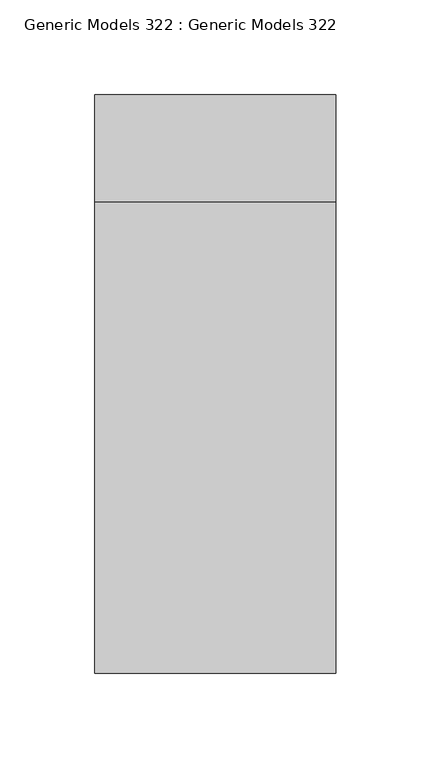
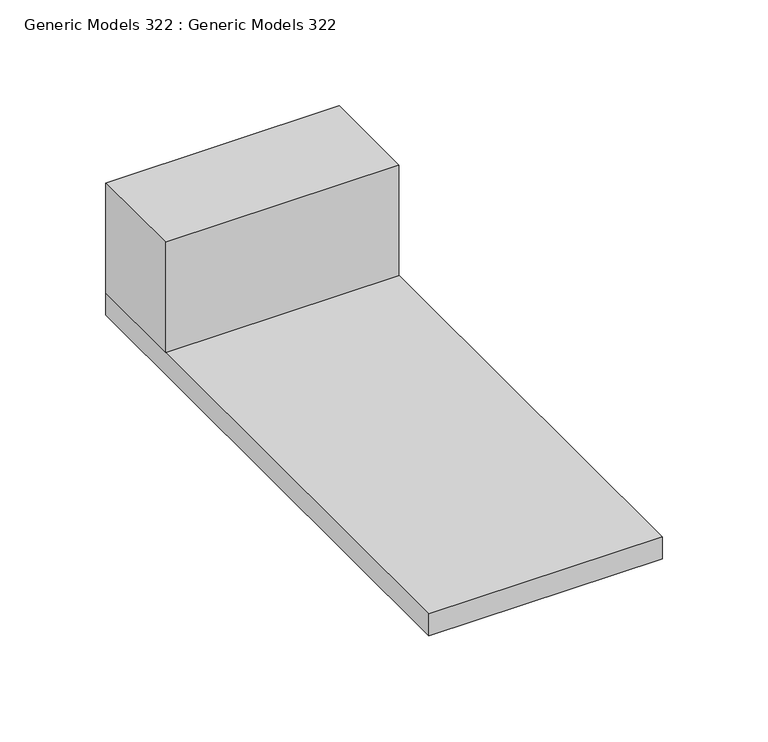
"""IFC4 building model written with IfcOpenShell, lengths in millimetres: proxy geometry, Generic Models 322 : Generic Models 322."""

from ifc_helpers import new_model, si_unit, frame, origin, place, context, project, spatial, polyline, outline, extrude, source, transform, mapped, element, save


def generic_models_322_generic_models_322_8154812b(model_context):
    return source(origin(), model_context, "Body", "SweptSolid", [
        extrude(outline(polyline([(1342.8513704, 704.5309662), (1469.8513704, 704.5309662), (1469.8513704, 648.1582392), (1342.8513704, 648.1582392), (1342.8513704, 704.5309662)])), frame((0.0, 0.0, 123310.396), z_axis=(0.0, 0.0, 1.0), x_axis=(1.0, 0.0, 0.0)), (0.0, 0.0, 1.0), 63.5),
        extrude(outline(polyline([(1342.8513704, 704.5309662), (1469.8513704, 704.5309662), (1469.8513704, 399.7309662), (1342.8513704, 399.7309662), (1342.8513704, 704.5309662)])), frame((0.0, 0.0, 123297.696), z_axis=(0.0, 0.0, 1.0), x_axis=(1.0, 0.0, 0.0)), (0.0, 0.0, 1.0), 12.7),
    ])


if __name__ == "__main__":
    model = new_model("IFC4")
    model_context = context("Model", 3, world=origin())
    ifc_project = project(units=[si_unit("LENGTHUNIT", "METRE", prefix="MILLI")], contexts=[model_context])
    site = spatial("IfcSite", under=ifc_project)
    building = spatial("IfcBuilding", under=site)
    placement = place(None, origin())
    generic_models_322_generic_models_322_shape = generic_models_322_generic_models_322_8154812b(model_context)
    element("IfcBuildingElementProxy", 1, Name="Generic Models 322 : Generic Models 322", ObjectType="Generic Models 322 : Generic Models 322", at=placement, inside=building, context=model_context, shape_type="MappedRepresentation", body=[
        mapped(generic_models_322_generic_models_322_shape, transform((0.0, 0.0, 0.0), x_axis=(1.0, 0.0, 0.0), y_axis=(0.0, 1.0, 0.0), z_axis=(0.0, 0.0, 1.0))),
    ])
    save(model, "model.ifc")

# Revit data of these elements
# Element 1 (IfcBuildingElementProxy, "Generic Models 322 : Generic Models 322")
#   Materials on its faces: "_HL35 EACH SIDE - SEE STRUCTURAL"
# Materials
#   "_HL35 EACH SIDE - SEE STRUCTURAL": class "Metal", colour RGB 199 199 199, transparency 0, Description = "Structural steel 50ksi", Cost = 0
